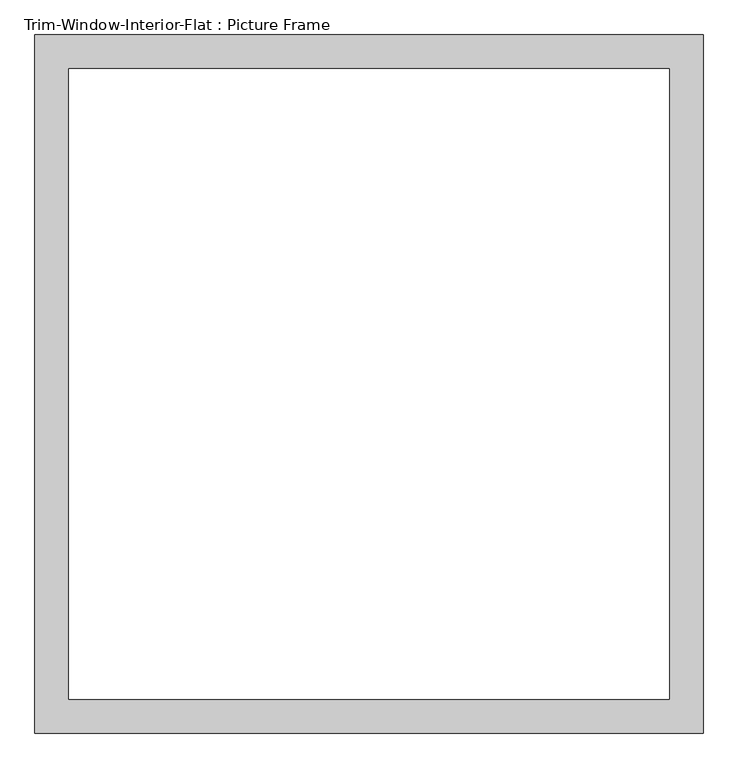
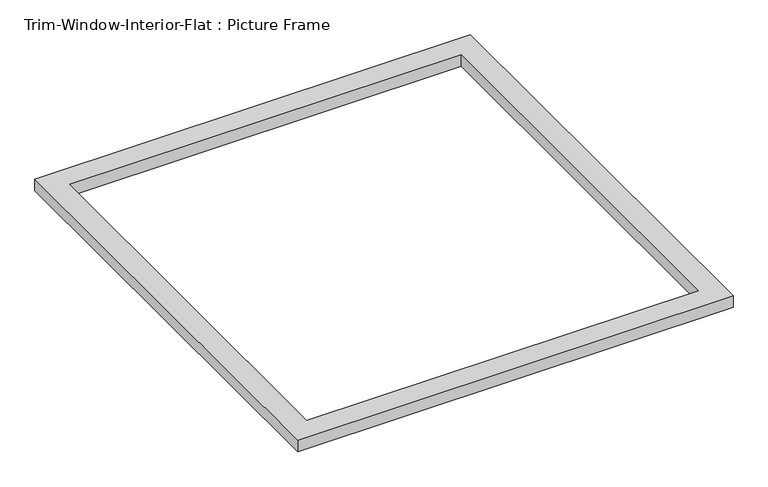
"""IFC4 building model written with IfcOpenShell, lengths in millimetres: proxy geometry, Trim-Window-Interior-Flat : Picture Frame."""

import ifcopenshell
import ifcopenshell.guid

model = None  # the IFC model being written
_history = None  # IfcOwnerHistory: only IFC2X3 demands one
_inside = {}  # id of a spatial element -> (the spatial element, [elements in it])
_under = {}  # id of a project, library or spatial element -> (it, [spatial elements below it])
_declared = {}  # id of a project -> (the project, [libraries it declares])
_typed = {}  # id of a type object -> (the type object, [elements of that type])
_made_of = {}  # id of a material, layer set ... -> (it, [elements and type objects made of it])


def new_model(schema):
    """Start an empty IFC model of exactly this schema.

    Asked for "IFC4X3", IfcOpenShell would pick the latest addendum, in which some entities
    have other attributes; the version numbers below select the first issue.
    IFC2X3 requires an IfcOwnerHistory on every rooted entity: one is made here for all.
    """
    global model, _history
    if schema == "IFC4X3":
        model = ifcopenshell.file(schema_version=(4, 3, 0, 0))
    else:
        model = ifcopenshell.file(schema=schema)
    _inside.clear()
    _under.clear()
    _declared.clear()
    _typed.clear()
    _made_of.clear()
    _history = None
    if model.schema == "IFC2X3":
        org = make("IfcOrganization", Name="unknown")
        user = make(
            "IfcPersonAndOrganization",
            ThePerson=make("IfcPerson", FamilyName="unknown"),
            TheOrganization=org,
        )
        app = make(
            "IfcApplication",
            ApplicationDeveloper=org,
            Version="unknown",
            ApplicationFullName="unknown",
            ApplicationIdentifier="unknown",
        )
        _history = make(
            "IfcOwnerHistory",
            OwningUser=user,
            OwningApplication=app,
            ChangeAction="ADDED",
            CreationDate=0,
        )
    return model


def make(cls, **values):
    """One entity of the class cls with the attributes given. An attribute that is None is left unset."""
    return model.create_entity(
        cls, **{name: value for name, value in values.items() if value is not None}
    )


def rooted(cls, **values):
    """An entity with a GlobalId (a new one), such as an element, a storey or a relation."""
    return make(cls, GlobalId=ifcopenshell.guid.new(), OwnerHistory=_history, **values)


def si_unit(unit_type, name, prefix=None):
    """IfcSIUnit, for example si_unit("LENGTHUNIT", "METRE", prefix="MILLI")."""
    return make("IfcSIUnit", UnitType=unit_type, Prefix=prefix, Name=name)


def assignment(units):
    """IfcUnitAssignment: the units of a project."""
    return None if units is None else make("IfcUnitAssignment", Units=units)


def point(xyz):
    """IfcCartesianPoint."""
    return None if xyz is None else make("IfcCartesianPoint", Coordinates=xyz)


def direction(xyz):
    """IfcDirection."""
    return None if xyz is None else make("IfcDirection", DirectionRatios=xyz)


def frame(location, z_axis=None, x_axis=None):
    """IfcAxis2Placement3D, a coordinate frame: its origin and axes. An axis left out is left unset."""
    return make(
        "IfcAxis2Placement3D",
        Location=point(location),
        Axis=direction(z_axis),
        RefDirection=direction(x_axis),
    )


def origin():
    """The frame at (0, 0, 0) with its axes left unset."""
    return frame((0.0, 0.0, 0.0))


def origin_with_axes():
    """The frame at (0, 0, 0) with the z axis (0, 0, 1) and the x axis (1, 0, 0) written out."""
    return frame((0.0, 0.0, 0.0), z_axis=(0.0, 0.0, 1.0), x_axis=(1.0, 0.0, 0.0))


def place(relative_to, where):
    """IfcLocalPlacement: puts the frame where relative to a parent placement (None: the world)."""
    return make(
        "IfcLocalPlacement", PlacementRelTo=relative_to, RelativePlacement=where
    )


def context(
    kind, dimensions, precision=None, world=None, true_north=None, identifier=None
):
    """IfcGeometricRepresentationContext, for example the 3D "Model" context."""
    return make(
        "IfcGeometricRepresentationContext",
        ContextIdentifier=identifier,
        ContextType=kind,
        CoordinateSpaceDimension=dimensions,
        Precision=precision,
        WorldCoordinateSystem=world,
        TrueNorth=true_north,
    )


def project(units=None, contexts=None):
    """IfcProject with its units and contexts."""
    return rooted(
        "IfcProject",
        Name="project",
        RepresentationContexts=contexts,
        UnitsInContext=assignment(units),
    )


def spatial(cls, under=None, at=None, **own):
    """A site, building, storey or space (cls), placed at a placement, below another one or the project."""
    s = rooted(cls, ObjectPlacement=at, **own)
    if under is not None:
        _under.setdefault(under.id(), (under, []))[1].append(s)
    return s


def polyline(points):
    """IfcPolyline through the points."""
    return make("IfcPolyline", Points=[point(p) for p in points])


def outline(outer, holes=None, kind="AREA"):
    """IfcArbitraryClosedProfileDef: a profile drawn as a closed curve; with holes, ...WithVoids."""
    if holes is None:
        return make("IfcArbitraryClosedProfileDef", ProfileType=kind, OuterCurve=outer)
    return make(
        "IfcArbitraryProfileDefWithVoids",
        ProfileType=kind,
        OuterCurve=outer,
        InnerCurves=holes,
    )


def extrude(swept, where, along, depth):
    """IfcExtrudedAreaSolid: the profile swept, set in the frame where, extruded along a direction by depth."""
    return make(
        "IfcExtrudedAreaSolid",
        SweptArea=swept,
        Position=where,
        ExtrudedDirection=direction(along),
        Depth=depth,
    )


def shape(context_of_items, identifier, shape_type, items):
    """IfcShapeRepresentation: the items that make up one representation, for example the "Body"."""
    return make(
        "IfcShapeRepresentation",
        ContextOfItems=context_of_items,
        RepresentationIdentifier=identifier,
        RepresentationType=shape_type,
        Items=items,
    )


def source(mapping_origin, context_of_items, identifier, shape_type, items):
    """IfcRepresentationMap: a shape defined once, which mapped items show again and again."""
    return make(
        "IfcRepresentationMap",
        MappingOrigin=mapping_origin,
        MappedRepresentation=shape(context_of_items, identifier, shape_type, items),
    )


def transform(
    local_origin,
    x_axis=None,
    y_axis=None,
    z_axis=None,
    scale=None,
    scale2=None,
    scale3=None,
    uniform=True,
):
    """IfcCartesianTransformationOperator3D, or its non-uniform kind. x_axis, y_axis, z_axis: its Axis1, 2, 3."""
    if uniform:
        return make(
            "IfcCartesianTransformationOperator3D",
            Axis1=direction(x_axis),
            Axis2=direction(y_axis),
            LocalOrigin=point(local_origin),
            Scale=scale,
            Axis3=direction(z_axis),
        )
    return make(
        "IfcCartesianTransformationOperator3DnonUniform",
        Axis1=direction(x_axis),
        Axis2=direction(y_axis),
        LocalOrigin=point(local_origin),
        Scale=scale,
        Axis3=direction(z_axis),
        Scale2=scale2,
        Scale3=scale3,
    )


def mapped(mapping_source, mapping_target):
    """IfcMappedItem: shows the shape of a source again, moved by a transform."""
    return make(
        "IfcMappedItem", MappingSource=mapping_source, MappingTarget=mapping_target
    )


def made_of(thing, what):
    """Note that an element or type object is made of a material, layer set ...; save() writes the relation."""
    if what is not None:
        _made_of.setdefault(what.id(), (what, []))[1].append(thing)
    return thing


def element(
    cls,
    number,
    at=None,
    inside=None,
    cuts=None,
    type_object=None,
    material=None,
    context=None,
    identifier="Body",
    shape_type=None,
    held_by="IfcProductDefinitionShape",
    body=None,
    shapes=None,
    **own,
):
    """One element of the class cls, such as IfcWall. Its Tag is "e" and its number.

    at: its placement. inside: the storey or other place that contains it. cuts: it is an
    opening in that element (IfcRelVoidsElement). A single representation is given by context,
    identifier, shape_type and body (its items); several are given by shapes. held_by: the class
    of the entity that holds the representations. save() writes the other relations.
    """
    e = rooted(cls, Tag="e%d" % number, ObjectPlacement=at, **own)
    if body is not None:
        shapes = [shape(context, identifier, shape_type, body)]
    if shapes is not None:
        e.Representation = make(held_by, Representations=shapes)
    if inside is not None:
        _inside.setdefault(inside.id(), (inside, []))[1].append(e)
    if cuts is not None:
        rooted(
            "IfcRelVoidsElement", RelatingBuildingElement=cuts, RelatedOpeningElement=e
        )
    if type_object is not None:
        _typed.setdefault(type_object.id(), (type_object, []))[1].append(e)
    return made_of(e, material)


def aggregate(whole, parts):
    """IfcRelAggregates: a whole, such as a stair, and the parts it consists of."""
    return rooted("IfcRelAggregates", RelatingObject=whole, RelatedObjects=parts)


def save(model, path):
    """Write the relations noted so far, then the file.

    IfcRelAggregates (storeys below a building ...), IfcRelContainedInSpatialStructure (elements
    in a storey), IfcRelDefinesByType, IfcRelAssociatesMaterial and IfcRelDeclares: one each for
    every whole, place, type object, material and project.
    """
    for whole, parts in _under.values():
        aggregate(whole, parts)
    for where, things in _inside.values():
        rooted(
            "IfcRelContainedInSpatialStructure",
            RelatedElements=things,
            RelatingStructure=where,
        )
    for kind, things in _typed.values():
        rooted("IfcRelDefinesByType", RelatedObjects=things, RelatingType=kind)
    for what, things in _made_of.values():
        rooted("IfcRelAssociatesMaterial", RelatedObjects=things, RelatingMaterial=what)
    for by, libraries in _declared.values():
        rooted("IfcRelDeclares", RelatingContext=by, RelatedDefinitions=libraries)
    model.write(path)


def trim_window_interior_flat_picture_frame_d507ee0b(model_context):
    return source(origin(), model_context, "Body", "SweptSolid", [
        extrude(outline(polyline([(565.15, -44.45), (-565.15, -44.45), (-565.15, 1136.65), (565.15, 1136.65), (565.15, -44.45)]), holes=[polyline([(508.0, 12.7), (508.0, 1079.5), (-508.0, 1079.5), (-508.0, 12.7), (508.0, 12.7)])]), origin_with_axes(), (0.0, 0.0, 1.0), 31.75),
    ])


if __name__ == "__main__":
    model = new_model("IFC4")
    model_context = context("Model", 3, world=origin())
    ifc_project = project(units=[si_unit("LENGTHUNIT", "METRE", prefix="MILLI")], contexts=[model_context])
    site = spatial("IfcSite", under=ifc_project)
    building = spatial("IfcBuilding", under=site)
    placement = place(None, origin())
    trim_window_interior_flat_picture_frame_shape = trim_window_interior_flat_picture_frame_d507ee0b(model_context)
    element("IfcBuildingElementProxy", 1, Name="Trim-Window-Interior-Flat : Picture Frame", ObjectType="Trim-Window-Interior-Flat : Picture Frame", at=placement, inside=building, context=model_context, shape_type="MappedRepresentation", body=[
        mapped(trim_window_interior_flat_picture_frame_shape, transform((0.0, 0.0, 0.0), x_axis=(1.0, 0.0, 0.0), y_axis=(0.0, 1.0, 0.0), z_axis=(0.0, 0.0, 1.0))),
    ])
    save(model, "model.ifc")

# Revit data of these elements
# Type "Trim-Window-Interior-Flat : Picture Frame"
#   Trim Thickness_Picture Frame = 0' - 1 1/4"
#   Trim Width = 0' - 2 1/4"
#   Trim Thickness_with Sill = 0' - 0 3/4"
#   Sill Thickness = 0' - 1 1/4"
#   Opening Width [instance default] = 2' - 0"
#   Opening Height [instance default] = 3' - 0"
#   Default Elevation = 4' - 0"
#   Sill = no
#   Picture Frame = yes
#   Trim Material [instance default] = none
# Element 1 (IfcBuildingElementProxy, "Trim-Window-Interior-Flat : Picture Frame")
#   Opening Width = 3' - 5"
#   Opening Height = 3' - 7"
#   Trim Material = Wood - Stained
#   Materials on its faces: "Wood - Stained"
# Materials
#   "Wood - Stained": class "Wood", colour RGB 224 178 126, transparency 0, Cost = 0
